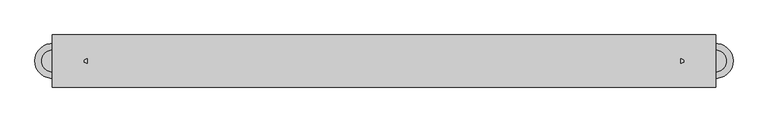
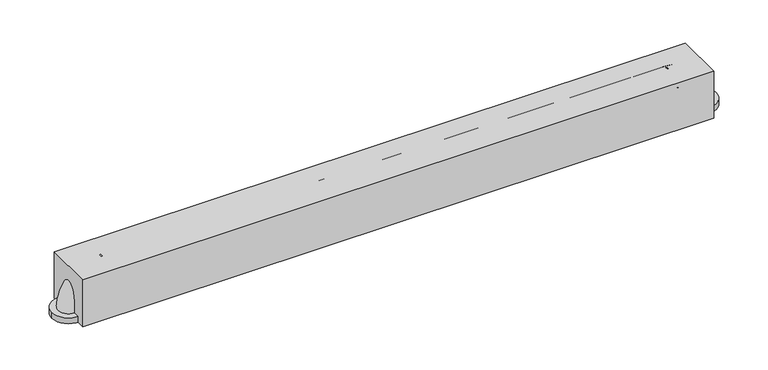
"""IFC4 building model written with IfcOpenShell, lengths in millimetres: proxy geometry, A5109 - Grab Bar, 1.25 in Dia, SS, 2 Wall, W-C Accessible : A5109 - Grab Bar, 1.25 in Dia, SS, 2 Wall, W-C Accessible."""

import ifcopenshell
import ifcopenshell.guid

model = None  # the IFC model being written
_history = None  # IfcOwnerHistory: only IFC2X3 demands one
_inside = {}  # id of a spatial element -> (the spatial element, [elements in it])
_under = {}  # id of a project, library or spatial element -> (it, [spatial elements below it])
_declared = {}  # id of a project -> (the project, [libraries it declares])
_typed = {}  # id of a type object -> (the type object, [elements of that type])
_made_of = {}  # id of a material, layer set ... -> (it, [elements and type objects made of it])


def new_model(schema):
    """Start an empty IFC model of exactly this schema.

    Asked for "IFC4X3", IfcOpenShell would pick the latest addendum, in which some entities
    have other attributes; the version numbers below select the first issue.
    IFC2X3 requires an IfcOwnerHistory on every rooted entity: one is made here for all.
    """
    global model, _history
    if schema == "IFC4X3":
        model = ifcopenshell.file(schema_version=(4, 3, 0, 0))
    else:
        model = ifcopenshell.file(schema=schema)
    _inside.clear()
    _under.clear()
    _declared.clear()
    _typed.clear()
    _made_of.clear()
    _history = None
    if model.schema == "IFC2X3":
        org = make("IfcOrganization", Name="unknown")
        user = make(
            "IfcPersonAndOrganization",
            ThePerson=make("IfcPerson", FamilyName="unknown"),
            TheOrganization=org,
        )
        app = make(
            "IfcApplication",
            ApplicationDeveloper=org,
            Version="unknown",
            ApplicationFullName="unknown",
            ApplicationIdentifier="unknown",
        )
        _history = make(
            "IfcOwnerHistory",
            OwningUser=user,
            OwningApplication=app,
            ChangeAction="ADDED",
            CreationDate=0,
        )
    return model


def make(cls, **values):
    """One entity of the class cls with the attributes given. An attribute that is None is left unset."""
    return model.create_entity(
        cls, **{name: value for name, value in values.items() if value is not None}
    )


def rooted(cls, **values):
    """An entity with a GlobalId (a new one), such as an element, a storey or a relation."""
    return make(cls, GlobalId=ifcopenshell.guid.new(), OwnerHistory=_history, **values)


def si_unit(unit_type, name, prefix=None):
    """IfcSIUnit, for example si_unit("LENGTHUNIT", "METRE", prefix="MILLI")."""
    return make("IfcSIUnit", UnitType=unit_type, Prefix=prefix, Name=name)


def assignment(units):
    """IfcUnitAssignment: the units of a project."""
    return None if units is None else make("IfcUnitAssignment", Units=units)


def point(xyz):
    """IfcCartesianPoint."""
    return None if xyz is None else make("IfcCartesianPoint", Coordinates=xyz)


def direction(xyz):
    """IfcDirection."""
    return None if xyz is None else make("IfcDirection", DirectionRatios=xyz)


def frame(location, z_axis=None, x_axis=None):
    """IfcAxis2Placement3D, a coordinate frame: its origin and axes. An axis left out is left unset."""
    return make(
        "IfcAxis2Placement3D",
        Location=point(location),
        Axis=direction(z_axis),
        RefDirection=direction(x_axis),
    )


def frame_2d(location, x_axis=None):
    """IfcAxis2Placement2D, a coordinate frame in the plane: its origin and x axis."""
    return make(
        "IfcAxis2Placement2D", Location=point(location), RefDirection=direction(x_axis)
    )


def origin():
    """The frame at (0, 0, 0) with its axes left unset."""
    return frame((0.0, 0.0, 0.0))


def origin_with_axes():
    """The frame at (0, 0, 0) with the z axis (0, 0, 1) and the x axis (1, 0, 0) written out."""
    return frame((0.0, 0.0, 0.0), z_axis=(0.0, 0.0, 1.0), x_axis=(1.0, 0.0, 0.0))


def place(relative_to, where):
    """IfcLocalPlacement: puts the frame where relative to a parent placement (None: the world)."""
    return make(
        "IfcLocalPlacement", PlacementRelTo=relative_to, RelativePlacement=where
    )


def context(
    kind, dimensions, precision=None, world=None, true_north=None, identifier=None
):
    """IfcGeometricRepresentationContext, for example the 3D "Model" context."""
    return make(
        "IfcGeometricRepresentationContext",
        ContextIdentifier=identifier,
        ContextType=kind,
        CoordinateSpaceDimension=dimensions,
        Precision=precision,
        WorldCoordinateSystem=world,
        TrueNorth=true_north,
    )


def project(units=None, contexts=None):
    """IfcProject with its units and contexts."""
    return rooted(
        "IfcProject",
        Name="project",
        RepresentationContexts=contexts,
        UnitsInContext=assignment(units),
    )


def spatial(cls, under=None, at=None, **own):
    """A site, building, storey or space (cls), placed at a placement, below another one or the project."""
    s = rooted(cls, ObjectPlacement=at, **own)
    if under is not None:
        _under.setdefault(under.id(), (under, []))[1].append(s)
    return s


def polyline(points):
    """IfcPolyline through the points."""
    return make("IfcPolyline", Points=[point(p) for p in points])


def circle_curve(where, radius):
    """IfcCircle in the frame where."""
    return make("IfcCircle", Position=where, Radius=radius)


def ellipse_curve(where, semi_axis1, semi_axis2):
    """IfcEllipse in the frame where."""
    return make(
        "IfcEllipse", Position=where, SemiAxis1=semi_axis1, SemiAxis2=semi_axis2
    )


def trimmed(basis, trim1, trim2, sense, master):
    """IfcTrimmedCurve: the piece of a basis curve between two trims."""
    return make(
        "IfcTrimmedCurve",
        BasisCurve=basis,
        Trim1=trim1,
        Trim2=trim2,
        SenseAgreement=sense,
        MasterRepresentation=master,
    )


def segment(curve, same_sense, transition):
    """IfcCompositeCurveSegment."""
    return make(
        "IfcCompositeCurveSegment",
        Transition=transition,
        SameSense=same_sense,
        ParentCurve=curve,
    )


def composite_curve(segments, self_intersect=None):
    """IfcCompositeCurve: segments joined end to end."""
    return make("IfcCompositeCurve", Segments=segments, SelfIntersect=self_intersect)


def outline(outer, holes=None, kind="AREA"):
    """IfcArbitraryClosedProfileDef: a profile drawn as a closed curve; with holes, ...WithVoids."""
    if holes is None:
        return make("IfcArbitraryClosedProfileDef", ProfileType=kind, OuterCurve=outer)
    return make(
        "IfcArbitraryProfileDefWithVoids",
        ProfileType=kind,
        OuterCurve=outer,
        InnerCurves=holes,
    )


def extrude(swept, where, along, depth):
    """IfcExtrudedAreaSolid: the profile swept, set in the frame where, extruded along a direction by depth."""
    return make(
        "IfcExtrudedAreaSolid",
        SweptArea=swept,
        Position=where,
        ExtrudedDirection=direction(along),
        Depth=depth,
    )


def shape(context_of_items, identifier, shape_type, items):
    """IfcShapeRepresentation: the items that make up one representation, for example the "Body"."""
    return make(
        "IfcShapeRepresentation",
        ContextOfItems=context_of_items,
        RepresentationIdentifier=identifier,
        RepresentationType=shape_type,
        Items=items,
    )


def source(mapping_origin, context_of_items, identifier, shape_type, items):
    """IfcRepresentationMap: a shape defined once, which mapped items show again and again."""
    return make(
        "IfcRepresentationMap",
        MappingOrigin=mapping_origin,
        MappedRepresentation=shape(context_of_items, identifier, shape_type, items),
    )


def transform(
    local_origin,
    x_axis=None,
    y_axis=None,
    z_axis=None,
    scale=None,
    scale2=None,
    scale3=None,
    uniform=True,
):
    """IfcCartesianTransformationOperator3D, or its non-uniform kind. x_axis, y_axis, z_axis: its Axis1, 2, 3."""
    if uniform:
        return make(
            "IfcCartesianTransformationOperator3D",
            Axis1=direction(x_axis),
            Axis2=direction(y_axis),
            LocalOrigin=point(local_origin),
            Scale=scale,
            Axis3=direction(z_axis),
        )
    return make(
        "IfcCartesianTransformationOperator3DnonUniform",
        Axis1=direction(x_axis),
        Axis2=direction(y_axis),
        LocalOrigin=point(local_origin),
        Scale=scale,
        Axis3=direction(z_axis),
        Scale2=scale2,
        Scale3=scale3,
    )


def mapped(mapping_source, mapping_target):
    """IfcMappedItem: shows the shape of a source again, moved by a transform."""
    return make(
        "IfcMappedItem", MappingSource=mapping_source, MappingTarget=mapping_target
    )


def made_of(thing, what):
    """Note that an element or type object is made of a material, layer set ...; save() writes the relation."""
    if what is not None:
        _made_of.setdefault(what.id(), (what, []))[1].append(thing)
    return thing


def element(
    cls,
    number,
    at=None,
    inside=None,
    cuts=None,
    type_object=None,
    material=None,
    context=None,
    identifier="Body",
    shape_type=None,
    held_by="IfcProductDefinitionShape",
    body=None,
    shapes=None,
    **own,
):
    """One element of the class cls, such as IfcWall. Its Tag is "e" and its number.

    at: its placement. inside: the storey or other place that contains it. cuts: it is an
    opening in that element (IfcRelVoidsElement). A single representation is given by context,
    identifier, shape_type and body (its items); several are given by shapes. held_by: the class
    of the entity that holds the representations. save() writes the other relations.
    """
    e = rooted(cls, Tag="e%d" % number, ObjectPlacement=at, **own)
    if body is not None:
        shapes = [shape(context, identifier, shape_type, body)]
    if shapes is not None:
        e.Representation = make(held_by, Representations=shapes)
    if inside is not None:
        _inside.setdefault(inside.id(), (inside, []))[1].append(e)
    if cuts is not None:
        rooted(
            "IfcRelVoidsElement", RelatingBuildingElement=cuts, RelatedOpeningElement=e
        )
    if type_object is not None:
        _typed.setdefault(type_object.id(), (type_object, []))[1].append(e)
    return made_of(e, material)


def aggregate(whole, parts):
    """IfcRelAggregates: a whole, such as a stair, and the parts it consists of."""
    return rooted("IfcRelAggregates", RelatingObject=whole, RelatedObjects=parts)


def save(model, path):
    """Write the relations noted so far, then the file.

    IfcRelAggregates (storeys below a building ...), IfcRelContainedInSpatialStructure (elements
    in a storey), IfcRelDefinesByType, IfcRelAssociatesMaterial and IfcRelDeclares: one each for
    every whole, place, type object, material and project.
    """
    for whole, parts in _under.values():
        aggregate(whole, parts)
    for where, things in _inside.values():
        rooted(
            "IfcRelContainedInSpatialStructure",
            RelatedElements=things,
            RelatingStructure=where,
        )
    for kind, things in _typed.values():
        rooted("IfcRelDefinesByType", RelatedObjects=things, RelatingType=kind)
    for what, things in _made_of.values():
        rooted("IfcRelAssociatesMaterial", RelatedObjects=things, RelatingMaterial=what)
    for by, libraries in _declared.values():
        rooted("IfcRelDeclares", RelatingContext=by, RelatedDefinitions=libraries)
    model.write(path)


def plane_surface(at):
    """IfcPlane: the flat surface through the origin of the frame at, square to its z axis."""
    return make("IfcPlane", Position=at)


def revolved_surface(curve, axis_point, axis_direction):
    """IfcSurfaceOfRevolution: the curve turned about the line through axis_point along axis_direction."""
    return make(
        "IfcSurfaceOfRevolution",
        SweptCurve=make("IfcArbitraryOpenProfileDef", ProfileType="CURVE", Curve=curve),
        AxisPosition=make("IfcAxis1Placement", Location=point(axis_point), Axis=direction(axis_direction)),
    )


def advanced_brep(points, edges, surfaces, faces):
    """IfcAdvancedBrep: a solid bounded by faces that lie on surfaces and meet in shared edges.

    An edge is (start, end): straight between two places in points (the first is 0);
    or (start, end, curve); or (start, end, curve, False) where it runs against its curve.
    A face is (place in surfaces, loops), or (place, loops, False) where it looks against
    its surface's normal. A loop lists edges by number (the first is 1), with a minus sign
    where the edge is run from its end to its start. The first loop is the outer one.
    """
    corners = [point(p) for p in points]
    vertices = [make("IfcVertexPoint", VertexGeometry=c) for c in corners]
    made = []
    for start, end, *more in edges:
        made.append(
            make(
                "IfcEdgeCurve",
                EdgeStart=vertices[start],
                EdgeEnd=vertices[end],
                EdgeGeometry=more[0] if more else make("IfcPolyline", Points=[corners[start], corners[end]]),
                SameSense=more[1] if len(more) > 1 else True,
            )
        )
    hull = []
    for where, loops, *sense in faces:
        bounds = []
        for j, loop in enumerate(loops):
            ring = [make("IfcOrientedEdge", EdgeElement=made[abs(k) - 1], Orientation=k > 0) for k in loop]
            bounds.append(
                make(
                    "IfcFaceOuterBound" if j == 0 else "IfcFaceBound",
                    Bound=make("IfcEdgeLoop", EdgeList=ring),
                    Orientation=True,
                )
            )
        hull.append(make("IfcAdvancedFace", Bounds=bounds, FaceSurface=surfaces[where], SameSense=sense[0] if sense else True))
    return make("IfcAdvancedBrep", Outer=make("IfcClosedShell", CfsFaces=hull))


def specialty_equipment_91fd0b1d(model_context):
    return source(origin(), model_context, "Body", "SolidModel", [
        advanced_brep(
        [(434.2435861, 15.875, 60.325), (434.2435861, -15.875, 60.325), (485.0435861, 15.875, 9.525), (485.0435861, -15.875, 9.525)],
        [
            (0, 1, circle_curve(frame((434.2435861, 0.0, 60.325), z_axis=(-1.0, 0.0, 0.0), x_axis=(0.0, -1.0, 0.0)), 15.875)),
            (1, 0, circle_curve(frame((434.2435861, 0.0, 60.325), z_axis=(-1.0, 0.0, 0.0), x_axis=(0.0, -1.0, 0.0)), 15.875)),
            (2, 3, circle_curve(frame((485.0435861, 0.0, 9.525), z_axis=(0.0, 0.0, -1.0), x_axis=(0.0, -1.0, 0.0)), 15.875)),
            (3, 2, circle_curve(frame((485.0435861, 0.0, 9.525), z_axis=(0.0, 0.0, -1.0), x_axis=(0.0, -1.0, 0.0)), 15.875)),
            (2, 0, circle_curve(frame((434.2435861, 15.875, 9.525), z_axis=(0.0, -1.0, 0.0), x_axis=(0.0, 0.0, 1.0)), 50.8)),
            (1, 3, circle_curve(frame((434.2435861, -15.875, 9.525), z_axis=(0.0, 1.0, 0.0), x_axis=(0.0, 0.0, 1.0)), 50.8)),
        ],
        [
            plane_surface(frame((434.2435861, 0.0, 60.325), z_axis=(-1.0, 0.0, 0.0), x_axis=(0.0, -1.0, 0.0))),
            plane_surface(frame((485.0435861, 0.0, 9.525), z_axis=(0.0, 0.0, -1.0), x_axis=(0.0, -1.0, 0.0))),
            revolved_surface(trimmed(ellipse_curve(frame((434.2435861, 0.0, 60.325), z_axis=(1.0, 0.0, 0.0), x_axis=(0.0, -1.0, 0.0)), 15.875, 15.875), [point((434.2435861, 15.875, 60.325))], [point((434.2435861, -15.875, 60.325))], True, "CARTESIAN"), (434.2435861, 0.0, 9.525), (0.0, -1.0, 0.0)),
            revolved_surface(trimmed(ellipse_curve(frame((434.2435861, 0.0, 60.325), z_axis=(1.0, 0.0, 0.0), x_axis=(0.0, -1.0, 0.0)), 15.875, 15.875), [point((434.2435861, -15.875, 60.325))], [point((434.2435861, 15.875, 60.325))], True, "CARTESIAN"), (434.2435861, 0.0, 9.525), (0.0, -1.0, 0.0)),
        ],
        [
            (0, [[1, 2]]),
            (1, [[3, 4]]),
            (2, [[-3, 5, -2, 6]]),
            (3, [[-4, -6, -1, -5]]),
        ],
    ),
        extrude(outline(composite_curve([segment(trimmed(circle_curve(frame_2d((485.0435861, 0.0)), 25.4), [point((510.4435861, 0.0))], [point((459.6435861, 0.0))], False, "CARTESIAN"), True, "CONTINUOUS"), segment(trimmed(circle_curve(frame_2d((485.0435861, 0.0)), 25.4), [point((459.6435861, 0.0))], [point((510.4435861, 0.0))], False, "CARTESIAN"), True, "CONTINUOUS")], self_intersect=False)), origin_with_axes(), (0.0, 0.0, 1.0), 9.525),
        advanced_brep(
        [(-434.2435861, 15.875, 60.325), (-434.2435861, -15.875, 60.325), (-485.0435861, 15.875, 9.525), (-485.0435861, -15.875, 9.525)],
        [
            (0, 1, circle_curve(frame((-434.2435861, 0.0, 60.325), z_axis=(1.0, 0.0, 0.0), x_axis=(0.0, -1.0, 0.0)), 15.875)),
            (1, 0, circle_curve(frame((-434.2435861, 0.0, 60.325), z_axis=(1.0, 0.0, 0.0), x_axis=(0.0, -1.0, 0.0)), 15.875)),
            (2, 3, circle_curve(frame((-485.0435861, 0.0, 9.525), z_axis=(0.0, 0.0, -1.0), x_axis=(0.0, -1.0, 0.0)), 15.875)),
            (3, 2, circle_curve(frame((-485.0435861, 0.0, 9.525), z_axis=(0.0, 0.0, -1.0), x_axis=(0.0, -1.0, 0.0)), 15.875)),
            (3, 1, circle_curve(frame((-434.2435861, -15.875, 9.525), z_axis=(0.0, 1.0, 0.0), x_axis=(0.0, 0.0, 1.0)), 50.8)),
            (0, 2, circle_curve(frame((-434.2435861, 15.875, 9.525), z_axis=(0.0, -1.0, 0.0), x_axis=(0.0, 0.0, 1.0)), 50.8)),
        ],
        [
            plane_surface(frame((-434.2435861, 0.0, 60.325), z_axis=(1.0, 0.0, 0.0), x_axis=(0.0, -1.0, 0.0))),
            plane_surface(frame((-485.0435861, 0.0, 9.525), z_axis=(0.0, 0.0, -1.0), x_axis=(0.0, -1.0, 0.0))),
            revolved_surface(trimmed(ellipse_curve(frame((-434.2435861, 0.0, 60.325), z_axis=(1.0, 0.0, 0.0), x_axis=(0.0, -1.0, 0.0)), 15.875, 15.875), [point((-434.2435861, 15.875, 60.325))], [point((-434.2435861, -15.875, 60.325))], True, "CARTESIAN"), (-434.2435861, 0.0, 9.525), (0.0, -1.0, 0.0)),
            revolved_surface(trimmed(ellipse_curve(frame((-434.2435861, 0.0, 60.325), z_axis=(1.0, 0.0, 0.0), x_axis=(0.0, -1.0, 0.0)), 15.875, 15.875), [point((-434.2435861, -15.875, 60.325))], [point((-434.2435861, 15.875, 60.325))], True, "CARTESIAN"), (-434.2435861, 0.0, 9.525), (0.0, -1.0, 0.0)),
        ],
        [
            (0, [[1, 2]]),
            (1, [[3, 4]]),
            (2, [[5, -1, 6, -4]]),
            (3, [[-6, -2, -5, -3]]),
        ],
    ),
        extrude(outline(composite_curve([segment(trimmed(circle_curve(frame_2d((-485.0435861, 0.0)), 25.4), [point((-510.4435861, 0.0))], [point((-459.6435861, 0.0))], False, "CARTESIAN"), True, "CONTINUOUS"), segment(trimmed(circle_curve(frame_2d((-485.0435861, 0.0)), 25.4), [point((-459.6435861, 0.0))], [point((-510.4435861, 0.0))], False, "CARTESIAN"), True, "CONTINUOUS")], self_intersect=False)), origin_with_axes(), (0.0, 0.0, 1.0), 9.525),
        extrude(outline(polyline([(485.0435861, -38.1), (-485.0435861, -38.1), (-485.0435861, 38.1), (485.0435861, 38.1), (485.0435861, -38.1)])), origin_with_axes(), (0.0, 0.0, 1.0), 76.2),
        extrude(outline(composite_curve([segment(trimmed(circle_curve(frame_2d((0.0, 60.325)), 15.875), [point((-15.875, 60.325))], [point((15.875, 60.325))], False, "CARTESIAN"), True, "CONTINUOUS"), segment(trimmed(circle_curve(frame_2d((0.0, 60.325)), 15.875), [point((15.875, 60.325))], [point((-15.875, 60.325))], False, "CARTESIAN"), True, "CONTINUOUS")], self_intersect=False)), frame((-434.2435861, 0.0, 0.0), z_axis=(1.0, 0.0, 0.0), x_axis=(0.0, 1.0, 0.0)), (0.0, 0.0, 1.0), 868.4871723),
    ])


if __name__ == "__main__":
    model = new_model("IFC4")
    model_context = context("Model", 3, world=origin())
    ifc_project = project(units=[si_unit("LENGTHUNIT", "METRE", prefix="MILLI")], contexts=[model_context])
    site = spatial("IfcSite", under=ifc_project)
    building = spatial("IfcBuilding", under=site)
    placement = place(None, origin())
    specialty_equipment_shape = specialty_equipment_91fd0b1d(model_context)
    element("IfcBuildingElementProxy", 1, Name="A5109 - Grab Bar, 1.25 in Dia, SS, 2 Wall, W-C Accessible : A5109 - Grab Bar, 1.25 in Dia, SS, 2 Wall, W-C Accessible", ObjectType="A5109 - Grab Bar, 1.25 in Dia, SS, 2 Wall, W-C Accessible : A5109 - Grab Bar, 1.25 in Dia, SS, 2 Wall, W-C Accessible", at=placement, inside=building, context=model_context, shape_type="MappedRepresentation", body=[
        mapped(specialty_equipment_shape, transform((0.0, 0.0, 0.0), x_axis=(1.0, 0.0, 0.0), y_axis=(0.0, 1.0, 0.0), z_axis=(0.0, 0.0, 1.0))),
    ])
    save(model, "model.ifc")

# Revit data of these elements
# Type "A5109 - Grab Bar, 1.25 in Dia, SS, 2 Wall, W-C Accessible : A5109 - Grab Bar, 1.25 in Dia, SS, 2 Wall, W-C Accessible"
#   Watts2 = "0"
#   Watts1 = "0"
#   Unit_Issue = "EA"
#   UTIL_6_Misc = "-"
#   UTIL_5_NonMedGas = "-"
#   UTIL_4_MiscGas = "-"
#   UTIL_3_MedGas = "-"
#   UTIL_2_Elec = "-"
#   UTIL_1_WaterDrain = "-"
#   Nomenclature = "Grab Bar, 1-1/4\" Dia., SS, 2 Wall, W/C Accessible"
#   NSN = "6530"
#   Location [instance default] = ""
#   JSN = "A5109"
#   Fund_Source_VA = "-"
#   Fund_Source_Navy = "-"
#   Fund_Source_Army = "-"
#   Fund_Source_AF = "-"
#   ELEC_Volts2 = "0"
#   ELEC_Volts1 = "0"
#   ELEC_Phase2 = "0"
#   ELEC_Phase1 = "0"
#   ELEC_HertzSwitch = "0"
#   ELEC_HertzDependent = "0"
#   ELEC_Hertz = "0"
#   ELEC_Amps2 = "0"
#   ELEC_Amps1 = "0"
#   DetailDescription = "A 1-1/4\" diameter, satin finish stainless steel, peened gripping surface, 2 wall toilet stall/ room, grab bar with concealed mounting flanges.  Snap over flanges are provided to conceal mounting screws. A selection of mounting kits and concealed anchor devices are available from the manufacturers for different types of installations. Grab bar shall comply with barrier-free accessibility guidelines for structural strength. For typical water closet applications in toilet stalls and rooms where ADA (American''s With Disabilities Act) requirements must be met."
#   CAT_VA = "A"
#   CAT_Navy = "A"
#   CAT_IHS = "-"
#   CAT_Army = "A"
#   CAT_AF = "A"
#   BTUperhour = "0"
#   Weight_IP = 7
#   Default Elevation = 2' - 9"
#   DIM_Width_IP = 4' - 9"
#   DIM_Height_IP = 0' - 3"
#   DIM_Depth_IP = 0' - 3"
#   CustomLength [instance default] = 2' - 0"
# Element 1 (IfcBuildingElementProxy, "A5109 - Grab Bar, 1.25 in Dia, SS, 2 Wall, W-C Accessible : A5109 - Grab Bar, 1.25 in Dia, SS, 2 Wall, W-C Accessible")
#   Location = "TLTS2"
#   CustomLength = 3' - 2.19241"
#   Materials on its faces: "EquipSpace"
# Materials
#   "EquipSpace": class "Unassigned", colour RGB 221 217 195, transparency 0.5
